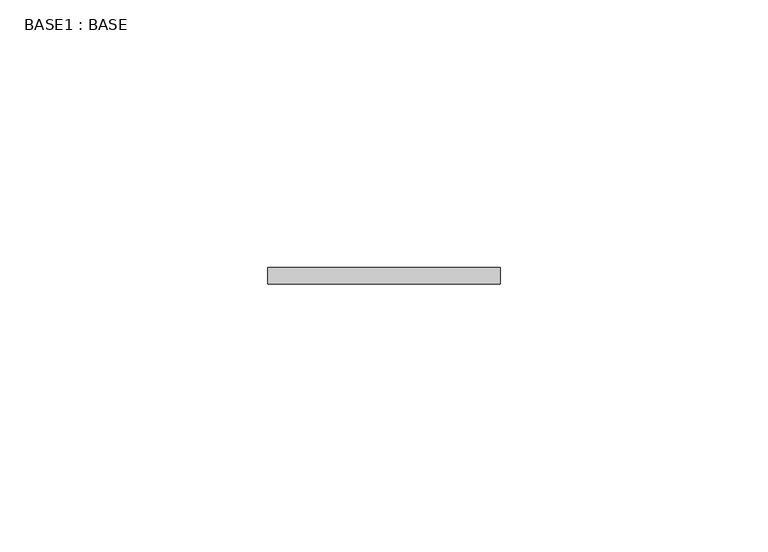
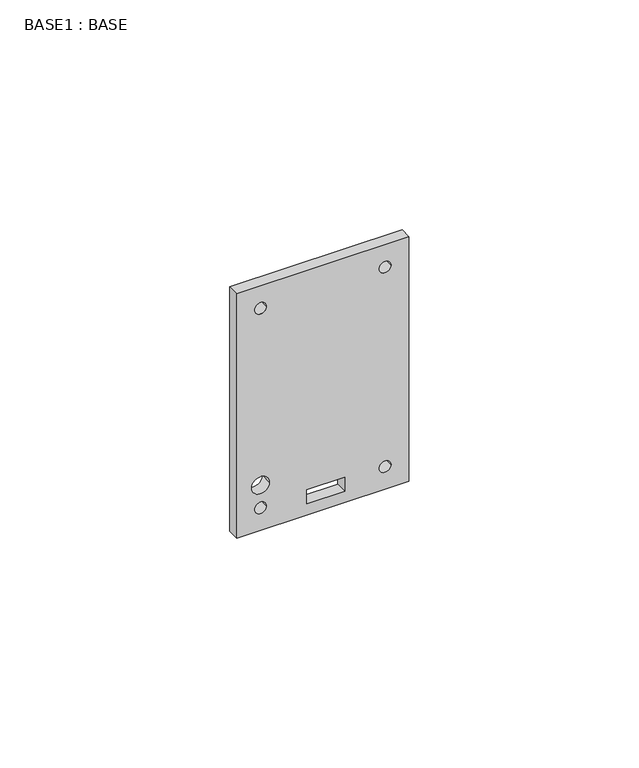
"""IFC4 building model written with IfcOpenShell, lengths in millimetres: proxy geometry, BASE1 : BASE."""

from ifc_helpers import new_model, si_unit, point, frame, frame_2d, origin, place, context, project, spatial, polyline, circle_curve, trimmed, segment, composite_curve, outline, extrude, source, transform, mapped, element, save


def base1_base_253a025e(model_context):
    return source(origin(), model_context, "Body", "SweptSolid", [
        extrude(outline(polyline([(0.0, 2369.0719295), (0.0, 2412.3719295), (65.0, 2412.3719295), (65.0, 2369.0719295), (0.0, 2369.0719295)]), holes=[composite_curve([segment(trimmed(circle_curve(frame_2d((59.0, 2406.3719295)), 1.5), [point((59.0, 2407.8719295))], [point((59.0, 2404.8719295))], True, "CARTESIAN"), True, "CONTINUOUS"), segment(trimmed(circle_curve(frame_2d((59.0, 2406.3719295)), 1.5), [point((59.0, 2404.8719295))], [point((59.0, 2407.8719295))], True, "CARTESIAN"), True, "CONTINUOUS")], self_intersect=False), composite_curve([segment(trimmed(circle_curve(frame_2d((59.0, 2375.0719295)), 1.5), [point((59.0, 2376.5719295))], [point((59.0, 2373.5719295))], True, "CARTESIAN"), True, "CONTINUOUS"), segment(trimmed(circle_curve(frame_2d((59.0, 2375.0719295)), 1.5), [point((59.0, 2373.5719295))], [point((59.0, 2376.5719295))], True, "CARTESIAN"), True, "CONTINUOUS")], self_intersect=False), composite_curve([segment(trimmed(circle_curve(frame_2d((6.0, 2375.0719295)), 1.5), [point((6.0, 2376.5719295))], [point((6.0, 2373.5719295))], True, "CARTESIAN"), True, "CONTINUOUS"), segment(trimmed(circle_curve(frame_2d((6.0, 2375.0719295)), 1.5), [point((6.0, 2373.5719295))], [point((6.0, 2376.5719295))], True, "CARTESIAN"), True, "CONTINUOUS")], self_intersect=False), composite_curve([segment(trimmed(circle_curve(frame_2d((6.0, 2406.3719295)), 1.5), [point((6.0, 2407.8719295))], [point((6.0, 2404.8719295))], True, "CARTESIAN"), True, "CONTINUOUS"), segment(trimmed(circle_curve(frame_2d((6.0, 2406.3719295)), 1.5), [point((6.0, 2404.8719295))], [point((6.0, 2407.8719295))], True, "CARTESIAN"), True, "CONTINUOUS")], self_intersect=False), composite_curve([segment(trimmed(circle_curve(frame_2d((12.0, 2375.0719295)), 2.25), [point((12.0, 2377.3219295))], [point((12.0, 2372.8219295))], True, "CARTESIAN"), True, "CONTINUOUS"), segment(trimmed(circle_curve(frame_2d((12.0, 2375.0719295)), 2.25), [point((12.0, 2372.8219295))], [point((12.0, 2377.3219295))], True, "CARTESIAN"), True, "CONTINUOUS")], self_intersect=False), polyline([(3.0, 2386.6931854), (6.75, 2386.6931854), (6.75, 2396.1931854), (3.0, 2396.1931854), (3.0, 2386.6931854)])]), frame((0.0, 1351.7384159, 0.0), z_axis=(0.0, 1.0, 0.0), x_axis=(0.0, 0.0, 1.0)), (0.0, 0.0, 1.0), 3.0),
    ])


if __name__ == "__main__":
    model = new_model("IFC4")
    model_context = context("Model", 3, world=origin())
    ifc_project = project(units=[si_unit("LENGTHUNIT", "METRE", prefix="MILLI")], contexts=[model_context])
    site = spatial("IfcSite", under=ifc_project)
    building = spatial("IfcBuilding", under=site)
    placement = place(None, origin())
    base1_base_shape = base1_base_253a025e(model_context)
    element("IfcBuildingElementProxy", 1, Name="BASE1 : BASE", ObjectType="BASE1 : BASE", at=placement, inside=building, context=model_context, shape_type="MappedRepresentation", body=[
        mapped(base1_base_shape, transform((0.0, 0.0, 0.0), x_axis=(1.0, 0.0, 0.0), y_axis=(0.0, 1.0, 0.0), z_axis=(0.0, 0.0, 1.0))),
    ])
    save(model, "model.ifc")

# Revit data of these elements
# Project information
#   Data de emissão do projeto = "Data de emissão"
#   Status do projeto = "Status do projeto"
#   Nome do cliente = "Proprietário"
#   Endereço do projeto = "Insira aqui o endereço"
#   Nome do projeto = "Nome do projeto"
#   Número do projeto = "0001"
# Element 1 (IfcBuildingElementProxy, "BASE1 : BASE")
#   Materials on its faces: ".BOX FUNDO"
# Materials
#   ".BOX FUNDO": class "Vidro", colour RGB 236 240 239, transparency 0.15, Cost = 0
